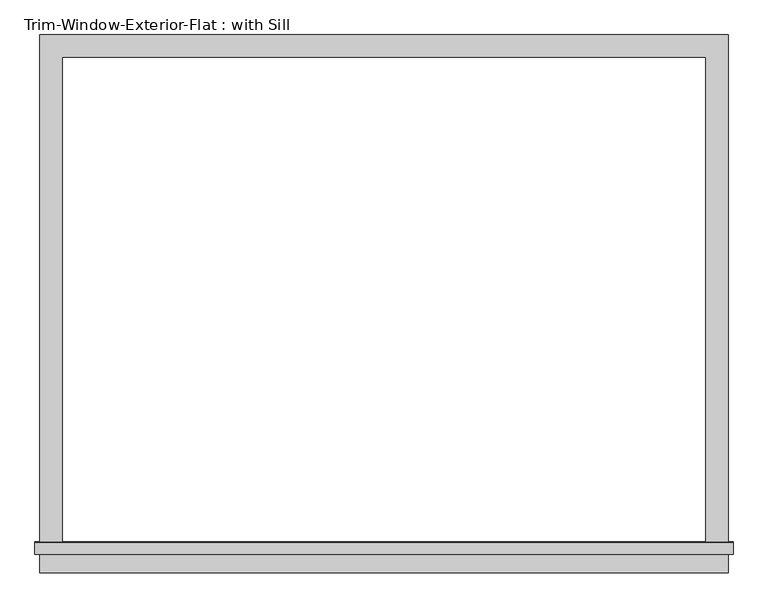
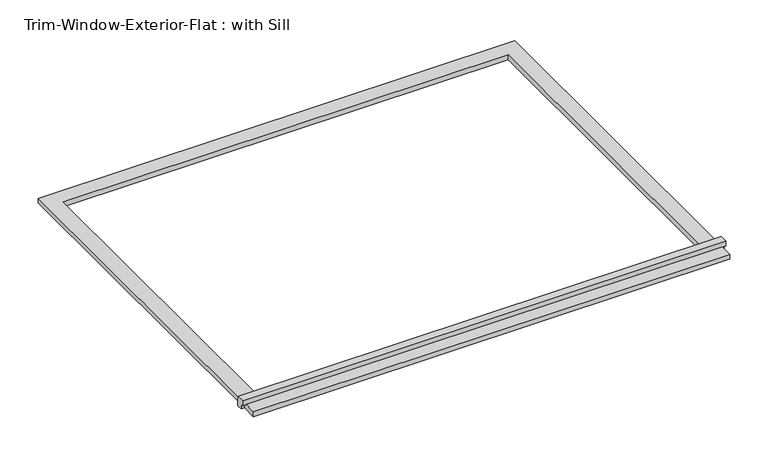
"""IFC4 building model written with IfcOpenShell, lengths in millimetres: proxy geometry, Trim-Window-Exterior-Flat : with Sill."""

import ifcopenshell
import ifcopenshell.guid

model = None  # the IFC model being written
_history = None  # IfcOwnerHistory: only IFC2X3 demands one
_inside = {}  # id of a spatial element -> (the spatial element, [elements in it])
_under = {}  # id of a project, library or spatial element -> (it, [spatial elements below it])
_declared = {}  # id of a project -> (the project, [libraries it declares])
_typed = {}  # id of a type object -> (the type object, [elements of that type])
_made_of = {}  # id of a material, layer set ... -> (it, [elements and type objects made of it])


def new_model(schema):
    """Start an empty IFC model of exactly this schema.

    Asked for "IFC4X3", IfcOpenShell would pick the latest addendum, in which some entities
    have other attributes; the version numbers below select the first issue.
    IFC2X3 requires an IfcOwnerHistory on every rooted entity: one is made here for all.
    """
    global model, _history
    if schema == "IFC4X3":
        model = ifcopenshell.file(schema_version=(4, 3, 0, 0))
    else:
        model = ifcopenshell.file(schema=schema)
    _inside.clear()
    _under.clear()
    _declared.clear()
    _typed.clear()
    _made_of.clear()
    _history = None
    if model.schema == "IFC2X3":
        org = make("IfcOrganization", Name="unknown")
        user = make(
            "IfcPersonAndOrganization",
            ThePerson=make("IfcPerson", FamilyName="unknown"),
            TheOrganization=org,
        )
        app = make(
            "IfcApplication",
            ApplicationDeveloper=org,
            Version="unknown",
            ApplicationFullName="unknown",
            ApplicationIdentifier="unknown",
        )
        _history = make(
            "IfcOwnerHistory",
            OwningUser=user,
            OwningApplication=app,
            ChangeAction="ADDED",
            CreationDate=0,
        )
    return model


def make(cls, **values):
    """One entity of the class cls with the attributes given. An attribute that is None is left unset."""
    return model.create_entity(
        cls, **{name: value for name, value in values.items() if value is not None}
    )


def rooted(cls, **values):
    """An entity with a GlobalId (a new one), such as an element, a storey or a relation."""
    return make(cls, GlobalId=ifcopenshell.guid.new(), OwnerHistory=_history, **values)


def si_unit(unit_type, name, prefix=None):
    """IfcSIUnit, for example si_unit("LENGTHUNIT", "METRE", prefix="MILLI")."""
    return make("IfcSIUnit", UnitType=unit_type, Prefix=prefix, Name=name)


def assignment(units):
    """IfcUnitAssignment: the units of a project."""
    return None if units is None else make("IfcUnitAssignment", Units=units)


def point(xyz):
    """IfcCartesianPoint."""
    return None if xyz is None else make("IfcCartesianPoint", Coordinates=xyz)


def direction(xyz):
    """IfcDirection."""
    return None if xyz is None else make("IfcDirection", DirectionRatios=xyz)


def frame(location, z_axis=None, x_axis=None):
    """IfcAxis2Placement3D, a coordinate frame: its origin and axes. An axis left out is left unset."""
    return make(
        "IfcAxis2Placement3D",
        Location=point(location),
        Axis=direction(z_axis),
        RefDirection=direction(x_axis),
    )


def origin():
    """The frame at (0, 0, 0) with its axes left unset."""
    return frame((0.0, 0.0, 0.0))


def origin_with_axes():
    """The frame at (0, 0, 0) with the z axis (0, 0, 1) and the x axis (1, 0, 0) written out."""
    return frame((0.0, 0.0, 0.0), z_axis=(0.0, 0.0, 1.0), x_axis=(1.0, 0.0, 0.0))


def place(relative_to, where):
    """IfcLocalPlacement: puts the frame where relative to a parent placement (None: the world)."""
    return make(
        "IfcLocalPlacement", PlacementRelTo=relative_to, RelativePlacement=where
    )


def context(
    kind, dimensions, precision=None, world=None, true_north=None, identifier=None
):
    """IfcGeometricRepresentationContext, for example the 3D "Model" context."""
    return make(
        "IfcGeometricRepresentationContext",
        ContextIdentifier=identifier,
        ContextType=kind,
        CoordinateSpaceDimension=dimensions,
        Precision=precision,
        WorldCoordinateSystem=world,
        TrueNorth=true_north,
    )


def project(units=None, contexts=None):
    """IfcProject with its units and contexts."""
    return rooted(
        "IfcProject",
        Name="project",
        RepresentationContexts=contexts,
        UnitsInContext=assignment(units),
    )


def spatial(cls, under=None, at=None, **own):
    """A site, building, storey or space (cls), placed at a placement, below another one or the project."""
    s = rooted(cls, ObjectPlacement=at, **own)
    if under is not None:
        _under.setdefault(under.id(), (under, []))[1].append(s)
    return s


def polyline(points):
    """IfcPolyline through the points."""
    return make("IfcPolyline", Points=[point(p) for p in points])


def outline(outer, holes=None, kind="AREA"):
    """IfcArbitraryClosedProfileDef: a profile drawn as a closed curve; with holes, ...WithVoids."""
    if holes is None:
        return make("IfcArbitraryClosedProfileDef", ProfileType=kind, OuterCurve=outer)
    return make(
        "IfcArbitraryProfileDefWithVoids",
        ProfileType=kind,
        OuterCurve=outer,
        InnerCurves=holes,
    )


def extrude(swept, where, along, depth):
    """IfcExtrudedAreaSolid: the profile swept, set in the frame where, extruded along a direction by depth."""
    return make(
        "IfcExtrudedAreaSolid",
        SweptArea=swept,
        Position=where,
        ExtrudedDirection=direction(along),
        Depth=depth,
    )


def shape(context_of_items, identifier, shape_type, items):
    """IfcShapeRepresentation: the items that make up one representation, for example the "Body"."""
    return make(
        "IfcShapeRepresentation",
        ContextOfItems=context_of_items,
        RepresentationIdentifier=identifier,
        RepresentationType=shape_type,
        Items=items,
    )


def source(mapping_origin, context_of_items, identifier, shape_type, items):
    """IfcRepresentationMap: a shape defined once, which mapped items show again and again."""
    return make(
        "IfcRepresentationMap",
        MappingOrigin=mapping_origin,
        MappedRepresentation=shape(context_of_items, identifier, shape_type, items),
    )


def transform(
    local_origin,
    x_axis=None,
    y_axis=None,
    z_axis=None,
    scale=None,
    scale2=None,
    scale3=None,
    uniform=True,
):
    """IfcCartesianTransformationOperator3D, or its non-uniform kind. x_axis, y_axis, z_axis: its Axis1, 2, 3."""
    if uniform:
        return make(
            "IfcCartesianTransformationOperator3D",
            Axis1=direction(x_axis),
            Axis2=direction(y_axis),
            LocalOrigin=point(local_origin),
            Scale=scale,
            Axis3=direction(z_axis),
        )
    return make(
        "IfcCartesianTransformationOperator3DnonUniform",
        Axis1=direction(x_axis),
        Axis2=direction(y_axis),
        LocalOrigin=point(local_origin),
        Scale=scale,
        Axis3=direction(z_axis),
        Scale2=scale2,
        Scale3=scale3,
    )


def mapped(mapping_source, mapping_target):
    """IfcMappedItem: shows the shape of a source again, moved by a transform."""
    return make(
        "IfcMappedItem", MappingSource=mapping_source, MappingTarget=mapping_target
    )


def made_of(thing, what):
    """Note that an element or type object is made of a material, layer set ...; save() writes the relation."""
    if what is not None:
        _made_of.setdefault(what.id(), (what, []))[1].append(thing)
    return thing


def element(
    cls,
    number,
    at=None,
    inside=None,
    cuts=None,
    type_object=None,
    material=None,
    context=None,
    identifier="Body",
    shape_type=None,
    held_by="IfcProductDefinitionShape",
    body=None,
    shapes=None,
    **own,
):
    """One element of the class cls, such as IfcWall. Its Tag is "e" and its number.

    at: its placement. inside: the storey or other place that contains it. cuts: it is an
    opening in that element (IfcRelVoidsElement). A single representation is given by context,
    identifier, shape_type and body (its items); several are given by shapes. held_by: the class
    of the entity that holds the representations. save() writes the other relations.
    """
    e = rooted(cls, Tag="e%d" % number, ObjectPlacement=at, **own)
    if body is not None:
        shapes = [shape(context, identifier, shape_type, body)]
    if shapes is not None:
        e.Representation = make(held_by, Representations=shapes)
    if inside is not None:
        _inside.setdefault(inside.id(), (inside, []))[1].append(e)
    if cuts is not None:
        rooted(
            "IfcRelVoidsElement", RelatingBuildingElement=cuts, RelatedOpeningElement=e
        )
    if type_object is not None:
        _typed.setdefault(type_object.id(), (type_object, []))[1].append(e)
    return made_of(e, material)


def aggregate(whole, parts):
    """IfcRelAggregates: a whole, such as a stair, and the parts it consists of."""
    return rooted("IfcRelAggregates", RelatingObject=whole, RelatedObjects=parts)


def save(model, path):
    """Write the relations noted so far, then the file.

    IfcRelAggregates (storeys below a building ...), IfcRelContainedInSpatialStructure (elements
    in a storey), IfcRelDefinesByType, IfcRelAssociatesMaterial and IfcRelDeclares: one each for
    every whole, place, type object, material and project.
    """
    for whole, parts in _under.values():
        aggregate(whole, parts)
    for where, things in _inside.values():
        rooted(
            "IfcRelContainedInSpatialStructure",
            RelatedElements=things,
            RelatingStructure=where,
        )
    for kind, things in _typed.values():
        rooted("IfcRelDefinesByType", RelatedObjects=things, RelatingType=kind)
    for what, things in _made_of.values():
        rooted("IfcRelAssociatesMaterial", RelatedObjects=things, RelatingMaterial=what)
    for by, libraries in _declared.values():
        rooted("IfcRelDeclares", RelatingContext=by, RelatedDefinitions=libraries)
    model.write(path)


def trim_window_exterior_flat_with_sill_12820e37(model_context):
    return source(origin(), model_context, "Body", "SweptSolid", [
        extrude(outline(polyline([(882.65, -1266.7823709), (882.65, -1323.9323709), (-882.65, -1323.9323709), (-882.65, -1266.7823709), (882.65, -1266.7823709)])), origin_with_axes(), (0.0, 0.0, 1.0), 19.05),
        extrude(outline(polyline([(-1276.35, 38.1), (-1247.0580645, 38.1), (-1244.6, 19.05), (-1244.6, 0.0), (-1266.7823709, 0.0), (-1266.7823709, 19.05), (-1276.35, 19.05), (-1276.35, 38.1)])), frame((-895.35, 0.0, 0.0), z_axis=(1.0, 0.0, 0.0), x_axis=(0.0, 1.0, 0.0)), (0.0, 0.0, 1.0), 1790.7),
        extrude(outline(polyline([(-882.65, 57.15), (882.65, 57.15), (882.65, -1244.6), (825.5, -1244.6), (825.5, 0.0), (-825.5, 0.0), (-825.5, -1244.6), (-882.65, -1244.6), (-882.65, 57.15)])), origin_with_axes(), (0.0, 0.0, 1.0), 19.05),
    ])


if __name__ == "__main__":
    model = new_model("IFC4")
    model_context = context("Model", 3, world=origin())
    ifc_project = project(units=[si_unit("LENGTHUNIT", "METRE", prefix="MILLI")], contexts=[model_context])
    site = spatial("IfcSite", under=ifc_project)
    building = spatial("IfcBuilding", under=site)
    placement = place(None, origin())
    trim_window_exterior_flat_with_sill_shape = trim_window_exterior_flat_with_sill_12820e37(model_context)
    element("IfcBuildingElementProxy", 1, Name="Trim-Window-Exterior-Flat : with Sill", ObjectType="Trim-Window-Exterior-Flat : with Sill", at=placement, inside=building, context=model_context, shape_type="MappedRepresentation", body=[
        mapped(trim_window_exterior_flat_with_sill_shape, transform((0.0, 0.0, 0.0), x_axis=(1.0, 0.0, 0.0), y_axis=(0.0, 1.0, 0.0), z_axis=(0.0, 0.0, 1.0))),
    ])
    save(model, "model.ifc")

# Revit data of these elements
# Project information
#   Project Issue Date = "09/11/2018"
#   Project Status = "Project Status"
#   Client Name = "Owner"
#   Project Address = "1021 HIGH ST -  MADISON, WI 53715"
#   Project Name = "2ND FLOOR ADDITION"
#   Project Number = "Project Number"
# Type "Trim-Window-Exterior-Flat : with Sill"
#   Trim Width = 0' - 2 1/4"
#   Trim Thickness_Picture Frame = 0' - 1 1/4"
#   Trim Thickness_with Sill = 0' - 0 3/4"
#   Sill Thickness = 0' - 1 1/4"
#   Opening Width [instance default] = 2' - 0"
#   Opening Height [instance default] = 3' - 0"
#   Default Elevation = 4' - 0"
#   Sill = yes
#   Picture Frame = no
#   Trim Material [instance default] = none
# Element 1 (IfcBuildingElementProxy, "Trim-Window-Exterior-Flat : with Sill")
#   Opening Width = 5' - 5"
#   Opening Height = 4' - 1"
#   Trim Material = Clad - White
#   Materials on its faces: "Clad - White"
# Materials
#   "Clad - White": class "Wood", colour RGB 242 242 238, transparency 0, Cost = 0
